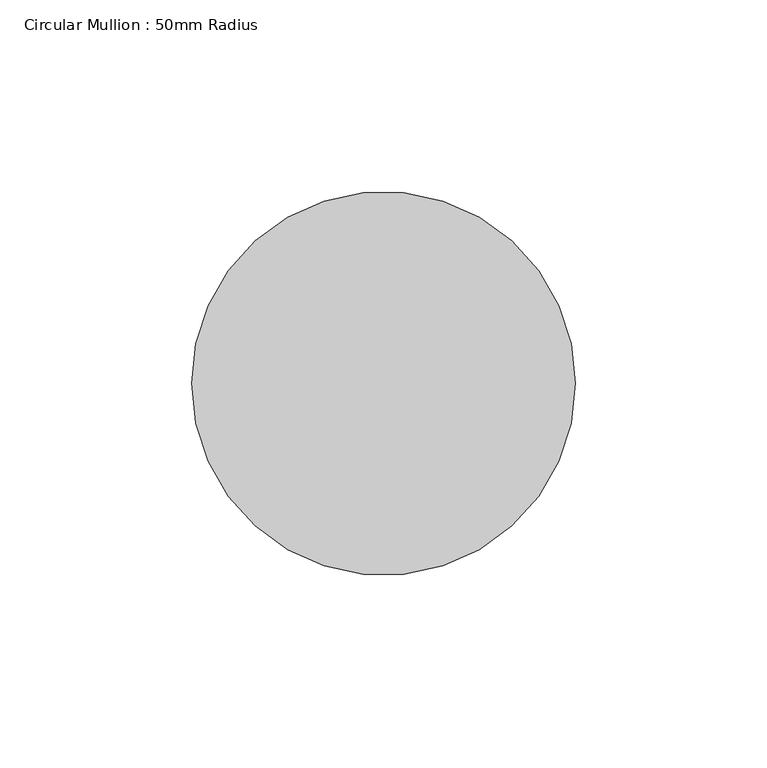
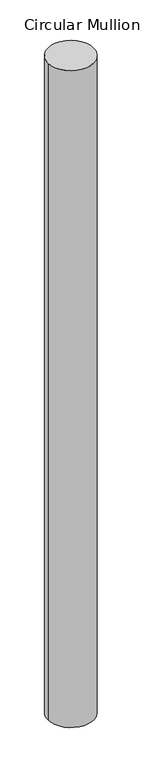
"""IFC4 building model written with IfcOpenShell, lengths in millimetres: member geometry, Circular Mullion : 50mm Radius."""

from ifc_helpers import new_model, si_unit, point, frame, origin, origin_2d, place, context, project, spatial, circle_curve, trimmed, segment, composite_curve, outline, extrude, source, transform, mapped, element, save


def circular_mullion_50mm_radius_4e59edd9(model_context):
    return source(origin(), model_context, "Body", "SweptSolid", [
        extrude(outline(composite_curve([segment(trimmed(circle_curve(origin_2d(), 50.0), [point((50.0, 0.0))], [point((-50.0, 0.0))], False, "CARTESIAN"), True, "CONTINUOUS"), segment(trimmed(circle_curve(origin_2d(), 50.0), [point((-50.0, 0.0))], [point((50.0, 0.0))], False, "CARTESIAN"), True, "CONTINUOUS")], self_intersect=False)), frame((0.0, 0.0, -1516.5918769), z_axis=(0.0, 0.0, 1.0), x_axis=(1.0, 0.0, 0.0)), (0.0, 0.0, 1.0), 1516.5918769),
    ])


if __name__ == "__main__":
    model = new_model("IFC4")
    model_context = context("Model", 3, world=origin())
    ifc_project = project(units=[si_unit("LENGTHUNIT", "METRE", prefix="MILLI")], contexts=[model_context])
    site = spatial("IfcSite", under=ifc_project)
    building = spatial("IfcBuilding", under=site)
    placement = place(None, origin())
    circular_mullion_50mm_radius_shape = circular_mullion_50mm_radius_4e59edd9(model_context)
    element("IfcMember", 1, ObjectType="Circular Mullion : 50mm Radius", at=placement, inside=building, context=model_context, shape_type="MappedRepresentation", body=[
        mapped(circular_mullion_50mm_radius_shape, transform((0.0, 0.0, 0.0), x_axis=(1.0, 0.0, 0.0), y_axis=(0.0, 1.0, 0.0), z_axis=(0.0, 0.0, 1.0))),
    ])
    save(model, "model.ifc")

# Revit data of these elements
# Type "Circular Mullion : 50mm Radius"
#   built-in parameter 1007350 = 0.164042 (stored number, unit not read)
# Element 1 (IfcMember, "Circular Mullion : 50mm Radius")
#   Materials on its faces: "Aluminium"
# Materials
#   "Aluminium": class "Metal", colour RGB 247 247 247, transparency 0, Description = "Aluminium 6061", Cost = 0
